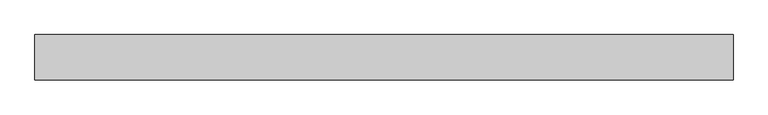
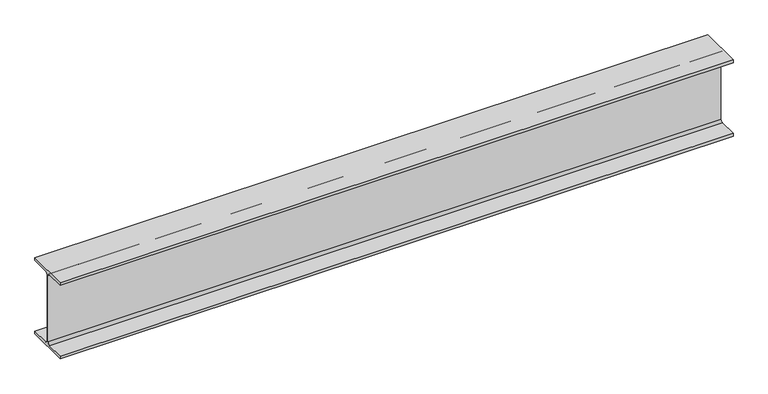
"""IFC4 building model written with IfcOpenShell, lengths in millimetres: beam geometry, Old_Steel Beam_H-KSD3502 : H_SB_ASB_H-350×175x7x11."""

from ifc_helpers import new_model, si_unit, point, frame, frame_2d, origin, place, context, project, spatial, polyline, circle_curve, trimmed, segment, composite_curve, outline, extrude, source, transform, mapped, element, save


def beam_87fd44ec(model_context):
    return source(origin(), model_context, "Body", "SweptSolid", [
        extrude(outline(composite_curve([segment(polyline([(82.5, -141.5), (82.5, -151.7), (-82.5, -151.7), (-82.5, -141.5), (-11.9, -141.5)]), True, "CONTINUOUS"), segment(trimmed(circle_curve(frame_2d((-11.9, -132.6)), 8.9), [point((-11.9, -141.5))], [point((-3.0, -132.6))], True, "CARTESIAN"), True, "CONTINUOUS"), segment(polyline([(-3.0, -132.6), (-3.0, 132.6)]), True, "CONTINUOUS"), segment(trimmed(circle_curve(frame_2d((-11.9, 132.6)), 8.9), [point((-3.0, 132.6))], [point((-11.9, 141.5))], True, "CARTESIAN"), True, "CONTINUOUS"), segment(polyline([(-11.9, 141.5), (-82.5, 141.5), (-82.5, 151.7), (82.5, 151.7), (82.5, 141.5), (11.9, 141.5)]), True, "CONTINUOUS"), segment(trimmed(circle_curve(frame_2d((11.9, 132.6)), 8.9), [point((11.9, 141.5))], [point((3.0, 132.6))], True, "CARTESIAN"), True, "CONTINUOUS"), segment(polyline([(3.0, 132.6), (3.0, -132.6)]), True, "CONTINUOUS"), segment(trimmed(circle_curve(frame_2d((11.9, -132.6)), 8.9), [point((3.0, -132.6))], [point((11.9, -141.5))], True, "CARTESIAN"), True, "CONTINUOUS"), segment(polyline([(11.9, -141.5), (82.5, -141.5)]), True, "CONTINUOUS")], self_intersect=False)), frame((-1244.2450896, 0.0, 0.0), z_axis=(1.0, 0.0, 0.0), x_axis=(0.0, 1.0, 0.0)), (0.0, 0.0, 1.0), 2540.0189947),
    ])


if __name__ == "__main__":
    model = new_model("IFC4")
    model_context = context("Model", 3, world=origin())
    ifc_project = project(units=[si_unit("LENGTHUNIT", "METRE", prefix="MILLI")], contexts=[model_context])
    site = spatial("IfcSite", under=ifc_project)
    building = spatial("IfcBuilding", under=site)
    placement = place(None, origin())
    beam_shape = beam_87fd44ec(model_context)
    element("IfcBeam", 1, ObjectType="Old_Steel Beam_H-KSD3502 : H_SB_ASB_H-350×175x7x11", at=placement, inside=building, context=model_context, shape_type="MappedRepresentation", body=[
        mapped(beam_shape, transform((0.0, 0.0, 0.0), x_axis=(1.0, 0.0, 0.0), y_axis=(0.0, 1.0, 0.0), z_axis=(0.0, 0.0, 1.0))),
    ])
    save(model, "model.ifc")

# Revit data of these elements
# Type "Old_Steel Beam_H-KSD3502 : H_SB_ASB_H-350×175x7x11"
#   Width = 17.5 cm
#   Web Thickness = 0.7 cm
#   Web Fillet = 1.4 cm
#   Warping Constant = 282290.0 cm⁶
#   Torsional Moment of Inertia = 19.4042 cm⁴
#   Torsional Modulus = 1.0 cm³
#   Section Area = 63.14 cm²
#   Plastic Modulus weak axis = 174.0 cm³
#   Plastic Modulus strong axis = 868.0 cm³
#   Perimeter = 1.36 m²/m
#   Nominal Weight = 49.60 kgf/m
#   Moment of Inertia weak axis = 984.00 cm⁴
#   Moment of Inertia strong axis = 13600.00 cm⁴
#   Height = 35.0 cm
#   Flange Thickness = 1.1 cm
#   Elastic Modulus weak axis = 112.0 cm³
#   Elastic Modulus strong axis = 775.0 cm³
#   Centroid Vertical = 17.5 cm
#   Centroid Horizontal = 8.75 cm
#   Length [instance default] = 1.5240 m
#   Structural Material [instance default] = Steel, 45-345
#   Assembly Code = ""
# Element 1 (IfcBeam, "Old_Steel Beam_H-KSD3502 : H_SB_ASB_H-350×175x7x11")
#   Structural Material = none
# Materials
#   "Steel, 45-345": class "Metal", colour RGB 189 187 185, transparency 0, Description = "Steel 345 MPa", Cost = 0
